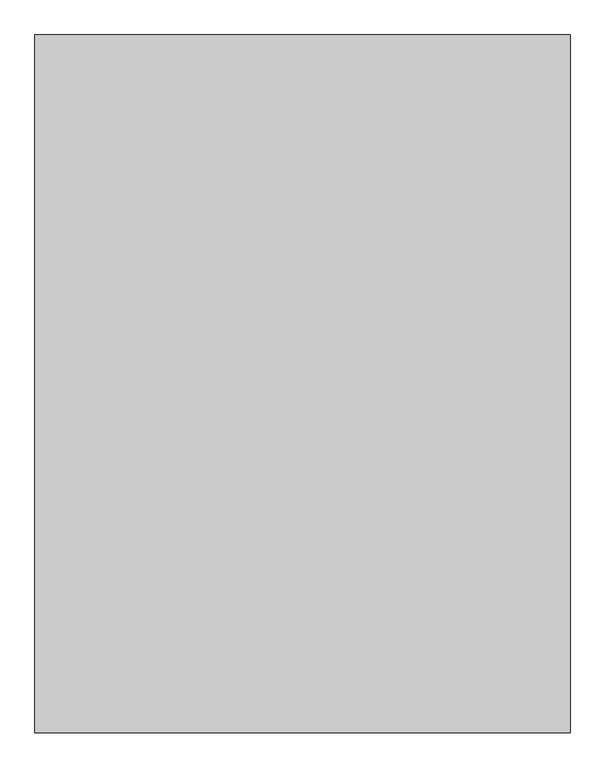
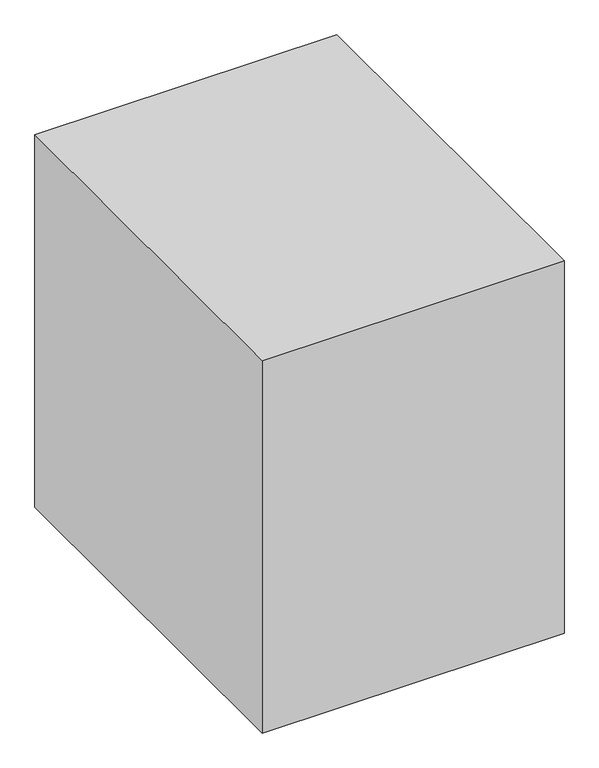
"""IFC4 building model written with IfcOpenShell, lengths in millimetres: proxy geometry, Space Planning Box_hec : Space Planning Box_hec."""

from ifc_helpers import new_model, si_unit, origin, origin_with_axes, place, context, project, spatial, polyline, outline, extrude, source, transform, mapped, element, save


def generic_models_1a87c0f4(model_context):
    return source(origin(), model_context, "Body", "SweptSolid", [
        extrude(outline(polyline([(2300.0, 3000.0), (2300.0, -3000.0), (-2300.0, -3000.0), (-2300.0, 3000.0), (2300.0, 3000.0)])), origin_with_axes(), (0.0, 0.0, 1.0), 6000.0),
    ])


if __name__ == "__main__":
    model = new_model("IFC4")
    model_context = context("Model", 3, world=origin())
    ifc_project = project(units=[si_unit("LENGTHUNIT", "METRE", prefix="MILLI")], contexts=[model_context])
    site = spatial("IfcSite", under=ifc_project)
    building = spatial("IfcBuilding", under=site)
    placement = place(None, origin())
    generic_models_shape = generic_models_1a87c0f4(model_context)
    element("IfcBuildingElementProxy", 1, Name="Space Planning Box_hec : Space Planning Box_hec", ObjectType="Space Planning Box_hec : Space Planning Box_hec", at=placement, inside=building, context=model_context, shape_type="MappedRepresentation", body=[
        mapped(generic_models_shape, transform((0.0, 0.0, 0.0), x_axis=(1.0, 0.0, 0.0), y_axis=(0.0, 1.0, 0.0), z_axis=(0.0, 0.0, 1.0))),
    ])
    save(model, "model.ifc")

# Revit data of these elements
# Type "Space Planning Box_hec : Space Planning Box_hec"
#   Type Comments = "..."
#   Room Name [instance default] = "?"
#   Interior Finish [instance default] = ""
#   Exterior Finish [instance default] = ""
#   Department [instance default] = ""
#   Assembly Code = "..."
#   Width [instance default] = 1524 mm
#   Program Area [instance default] = 0.00 m²
#   Length [instance default] = 1524 mm
#   Height [instance default] = 1524 mm
#   Area [instance default] = 2.32258 m²
#   Fill Color [instance default] = Cyan
#   Default Elevation = 0
# Element 1 (IfcBuildingElementProxy, "Space Planning Box_hec : Space Planning Box_hec")
#   Room Name = "Document Room"
#   Interior Finish = "IF2-1"
#   Exterior Finish = "EF1"
#   Department = "AR"
#   Width = 4600 mm
#   Program Area = 48.00 m²
#   Length = 6000 mm
#   Height = 6000 mm
#   Area = 27.60 m²
#   Fill Color = Lavender
#   Materials on its faces: "Lavender"
# Materials
#   "Cyan": class "Generic", colour RGB 0 255 255, transparency 0.2, Cost = 0
#   "Lavender": class "Generic", colour RGB 186 85 211, transparency 0.2, Cost = 0
